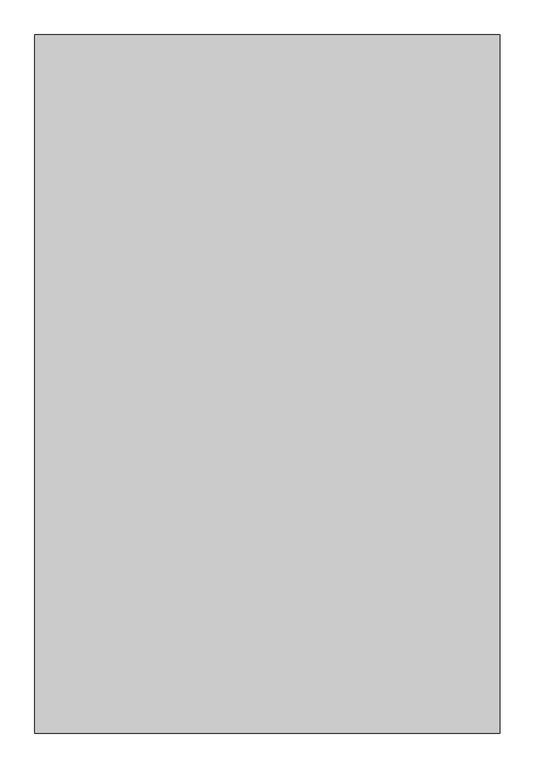
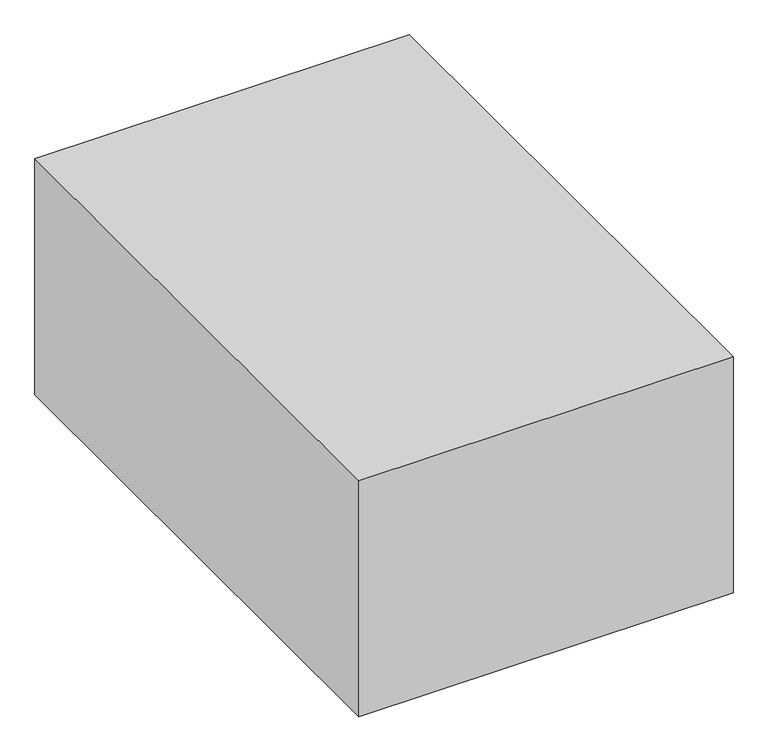
"""IFC4 building model written with IfcOpenShell, lengths in millimetres: proxy geometry, Space Planning Box_hec : Space Planning Box_hec."""

import ifcopenshell
import ifcopenshell.guid

model = None  # the IFC model being written
_history = None  # IfcOwnerHistory: only IFC2X3 demands one
_inside = {}  # id of a spatial element -> (the spatial element, [elements in it])
_under = {}  # id of a project, library or spatial element -> (it, [spatial elements below it])
_declared = {}  # id of a project -> (the project, [libraries it declares])
_typed = {}  # id of a type object -> (the type object, [elements of that type])
_made_of = {}  # id of a material, layer set ... -> (it, [elements and type objects made of it])


def new_model(schema):
    """Start an empty IFC model of exactly this schema.

    Asked for "IFC4X3", IfcOpenShell would pick the latest addendum, in which some entities
    have other attributes; the version numbers below select the first issue.
    IFC2X3 requires an IfcOwnerHistory on every rooted entity: one is made here for all.
    """
    global model, _history
    if schema == "IFC4X3":
        model = ifcopenshell.file(schema_version=(4, 3, 0, 0))
    else:
        model = ifcopenshell.file(schema=schema)
    _inside.clear()
    _under.clear()
    _declared.clear()
    _typed.clear()
    _made_of.clear()
    _history = None
    if model.schema == "IFC2X3":
        org = make("IfcOrganization", Name="unknown")
        user = make(
            "IfcPersonAndOrganization",
            ThePerson=make("IfcPerson", FamilyName="unknown"),
            TheOrganization=org,
        )
        app = make(
            "IfcApplication",
            ApplicationDeveloper=org,
            Version="unknown",
            ApplicationFullName="unknown",
            ApplicationIdentifier="unknown",
        )
        _history = make(
            "IfcOwnerHistory",
            OwningUser=user,
            OwningApplication=app,
            ChangeAction="ADDED",
            CreationDate=0,
        )
    return model


def make(cls, **values):
    """One entity of the class cls with the attributes given. An attribute that is None is left unset."""
    return model.create_entity(
        cls, **{name: value for name, value in values.items() if value is not None}
    )


def rooted(cls, **values):
    """An entity with a GlobalId (a new one), such as an element, a storey or a relation."""
    return make(cls, GlobalId=ifcopenshell.guid.new(), OwnerHistory=_history, **values)


def si_unit(unit_type, name, prefix=None):
    """IfcSIUnit, for example si_unit("LENGTHUNIT", "METRE", prefix="MILLI")."""
    return make("IfcSIUnit", UnitType=unit_type, Prefix=prefix, Name=name)


def assignment(units):
    """IfcUnitAssignment: the units of a project."""
    return None if units is None else make("IfcUnitAssignment", Units=units)


def point(xyz):
    """IfcCartesianPoint."""
    return None if xyz is None else make("IfcCartesianPoint", Coordinates=xyz)


def direction(xyz):
    """IfcDirection."""
    return None if xyz is None else make("IfcDirection", DirectionRatios=xyz)


def frame(location, z_axis=None, x_axis=None):
    """IfcAxis2Placement3D, a coordinate frame: its origin and axes. An axis left out is left unset."""
    return make(
        "IfcAxis2Placement3D",
        Location=point(location),
        Axis=direction(z_axis),
        RefDirection=direction(x_axis),
    )


def origin():
    """The frame at (0, 0, 0) with its axes left unset."""
    return frame((0.0, 0.0, 0.0))


def origin_with_axes():
    """The frame at (0, 0, 0) with the z axis (0, 0, 1) and the x axis (1, 0, 0) written out."""
    return frame((0.0, 0.0, 0.0), z_axis=(0.0, 0.0, 1.0), x_axis=(1.0, 0.0, 0.0))


def place(relative_to, where):
    """IfcLocalPlacement: puts the frame where relative to a parent placement (None: the world)."""
    return make(
        "IfcLocalPlacement", PlacementRelTo=relative_to, RelativePlacement=where
    )


def context(
    kind, dimensions, precision=None, world=None, true_north=None, identifier=None
):
    """IfcGeometricRepresentationContext, for example the 3D "Model" context."""
    return make(
        "IfcGeometricRepresentationContext",
        ContextIdentifier=identifier,
        ContextType=kind,
        CoordinateSpaceDimension=dimensions,
        Precision=precision,
        WorldCoordinateSystem=world,
        TrueNorth=true_north,
    )


def project(units=None, contexts=None):
    """IfcProject with its units and contexts."""
    return rooted(
        "IfcProject",
        Name="project",
        RepresentationContexts=contexts,
        UnitsInContext=assignment(units),
    )


def spatial(cls, under=None, at=None, **own):
    """A site, building, storey or space (cls), placed at a placement, below another one or the project."""
    s = rooted(cls, ObjectPlacement=at, **own)
    if under is not None:
        _under.setdefault(under.id(), (under, []))[1].append(s)
    return s


def polyline(points):
    """IfcPolyline through the points."""
    return make("IfcPolyline", Points=[point(p) for p in points])


def outline(outer, holes=None, kind="AREA"):
    """IfcArbitraryClosedProfileDef: a profile drawn as a closed curve; with holes, ...WithVoids."""
    if holes is None:
        return make("IfcArbitraryClosedProfileDef", ProfileType=kind, OuterCurve=outer)
    return make(
        "IfcArbitraryProfileDefWithVoids",
        ProfileType=kind,
        OuterCurve=outer,
        InnerCurves=holes,
    )


def extrude(swept, where, along, depth):
    """IfcExtrudedAreaSolid: the profile swept, set in the frame where, extruded along a direction by depth."""
    return make(
        "IfcExtrudedAreaSolid",
        SweptArea=swept,
        Position=where,
        ExtrudedDirection=direction(along),
        Depth=depth,
    )


def shape(context_of_items, identifier, shape_type, items):
    """IfcShapeRepresentation: the items that make up one representation, for example the "Body"."""
    return make(
        "IfcShapeRepresentation",
        ContextOfItems=context_of_items,
        RepresentationIdentifier=identifier,
        RepresentationType=shape_type,
        Items=items,
    )


def source(mapping_origin, context_of_items, identifier, shape_type, items):
    """IfcRepresentationMap: a shape defined once, which mapped items show again and again."""
    return make(
        "IfcRepresentationMap",
        MappingOrigin=mapping_origin,
        MappedRepresentation=shape(context_of_items, identifier, shape_type, items),
    )


def transform(
    local_origin,
    x_axis=None,
    y_axis=None,
    z_axis=None,
    scale=None,
    scale2=None,
    scale3=None,
    uniform=True,
):
    """IfcCartesianTransformationOperator3D, or its non-uniform kind. x_axis, y_axis, z_axis: its Axis1, 2, 3."""
    if uniform:
        return make(
            "IfcCartesianTransformationOperator3D",
            Axis1=direction(x_axis),
            Axis2=direction(y_axis),
            LocalOrigin=point(local_origin),
            Scale=scale,
            Axis3=direction(z_axis),
        )
    return make(
        "IfcCartesianTransformationOperator3DnonUniform",
        Axis1=direction(x_axis),
        Axis2=direction(y_axis),
        LocalOrigin=point(local_origin),
        Scale=scale,
        Axis3=direction(z_axis),
        Scale2=scale2,
        Scale3=scale3,
    )


def mapped(mapping_source, mapping_target):
    """IfcMappedItem: shows the shape of a source again, moved by a transform."""
    return make(
        "IfcMappedItem", MappingSource=mapping_source, MappingTarget=mapping_target
    )


def made_of(thing, what):
    """Note that an element or type object is made of a material, layer set ...; save() writes the relation."""
    if what is not None:
        _made_of.setdefault(what.id(), (what, []))[1].append(thing)
    return thing


def element(
    cls,
    number,
    at=None,
    inside=None,
    cuts=None,
    type_object=None,
    material=None,
    context=None,
    identifier="Body",
    shape_type=None,
    held_by="IfcProductDefinitionShape",
    body=None,
    shapes=None,
    **own,
):
    """One element of the class cls, such as IfcWall. Its Tag is "e" and its number.

    at: its placement. inside: the storey or other place that contains it. cuts: it is an
    opening in that element (IfcRelVoidsElement). A single representation is given by context,
    identifier, shape_type and body (its items); several are given by shapes. held_by: the class
    of the entity that holds the representations. save() writes the other relations.
    """
    e = rooted(cls, Tag="e%d" % number, ObjectPlacement=at, **own)
    if body is not None:
        shapes = [shape(context, identifier, shape_type, body)]
    if shapes is not None:
        e.Representation = make(held_by, Representations=shapes)
    if inside is not None:
        _inside.setdefault(inside.id(), (inside, []))[1].append(e)
    if cuts is not None:
        rooted(
            "IfcRelVoidsElement", RelatingBuildingElement=cuts, RelatedOpeningElement=e
        )
    if type_object is not None:
        _typed.setdefault(type_object.id(), (type_object, []))[1].append(e)
    return made_of(e, material)


def aggregate(whole, parts):
    """IfcRelAggregates: a whole, such as a stair, and the parts it consists of."""
    return rooted("IfcRelAggregates", RelatingObject=whole, RelatedObjects=parts)


def save(model, path):
    """Write the relations noted so far, then the file.

    IfcRelAggregates (storeys below a building ...), IfcRelContainedInSpatialStructure (elements
    in a storey), IfcRelDefinesByType, IfcRelAssociatesMaterial and IfcRelDeclares: one each for
    every whole, place, type object, material and project.
    """
    for whole, parts in _under.values():
        aggregate(whole, parts)
    for where, things in _inside.values():
        rooted(
            "IfcRelContainedInSpatialStructure",
            RelatedElements=things,
            RelatingStructure=where,
        )
    for kind, things in _typed.values():
        rooted("IfcRelDefinesByType", RelatedObjects=things, RelatingType=kind)
    for what, things in _made_of.values():
        rooted("IfcRelAssociatesMaterial", RelatedObjects=things, RelatingMaterial=what)
    for by, libraries in _declared.values():
        rooted("IfcRelDeclares", RelatingContext=by, RelatedDefinitions=libraries)
    model.write(path)


def generic_models_df3bc381(model_context):
    return source(origin(), model_context, "Body", "SweptSolid", [
        extrude(outline(polyline([(4500.0, 6750.0), (4500.0, -6750.0), (-4500.0, -6750.0), (-4500.0, 6750.0), (4500.0, 6750.0)])), origin_with_axes(), (0.0, 0.0, 1.0), 6000.0),
    ])


if __name__ == "__main__":
    model = new_model("IFC4")
    model_context = context("Model", 3, world=origin())
    ifc_project = project(units=[si_unit("LENGTHUNIT", "METRE", prefix="MILLI")], contexts=[model_context])
    site = spatial("IfcSite", under=ifc_project)
    building = spatial("IfcBuilding", under=site)
    placement = place(None, origin())
    generic_models_shape = generic_models_df3bc381(model_context)
    element("IfcBuildingElementProxy", 1, Name="Space Planning Box_hec : Space Planning Box_hec", ObjectType="Space Planning Box_hec : Space Planning Box_hec", at=placement, inside=building, context=model_context, shape_type="MappedRepresentation", body=[
        mapped(generic_models_shape, transform((0.0, 0.0, 0.0), x_axis=(1.0, 0.0, 0.0), y_axis=(0.0, 1.0, 0.0), z_axis=(0.0, 0.0, 1.0))),
    ])
    save(model, "model.ifc")

# Revit data of these elements
# Type "Space Planning Box_hec : Space Planning Box_hec"
#   Type Comments = "..."
#   Room Name [instance default] = "?"
#   Interior Finish [instance default] = ""
#   Exterior Finish [instance default] = ""
#   Department [instance default] = ""
#   Assembly Code = "..."
#   Width [instance default] = 1524 mm
#   Program Area [instance default] = 0.00 m²
#   Length [instance default] = 1524 mm
#   Height [instance default] = 1524 mm
#   Area [instance default] = 2.32258 m²
#   Fill Color [instance default] = Cyan
#   Default Elevation = 0
# Element 1 (IfcBuildingElementProxy, "Space Planning Box_hec : Space Planning Box_hec")
#   Room Name = "Engineer Room"
#   Interior Finish = "IF3"
#   Exterior Finish = "EF1"
#   Department = "CI"
#   Width = 9000 mm
#   Program Area = 120.00 m²
#   Length = 13500 mm
#   Height = 6000 mm
#   Area = 121.50 m²
#   Fill Color = Lime
#   Materials on its faces: "Lime"
# Materials
#   "Cyan": class "Generic", colour RGB 0 255 255, transparency 0.2, Cost = 0
#   "Lime": class "Generic", colour RGB 0 255 0, transparency 0.2, Cost = 0
